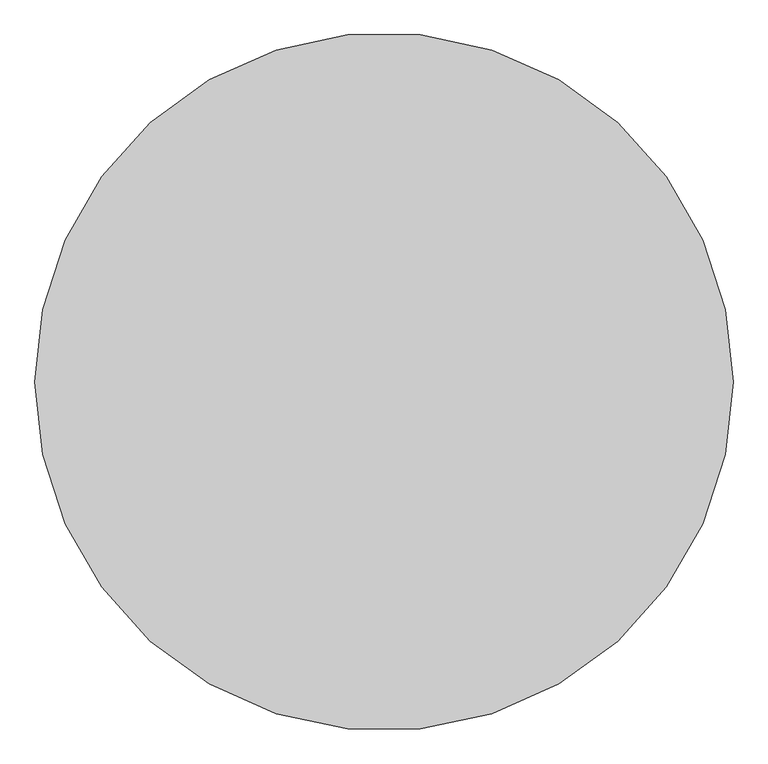
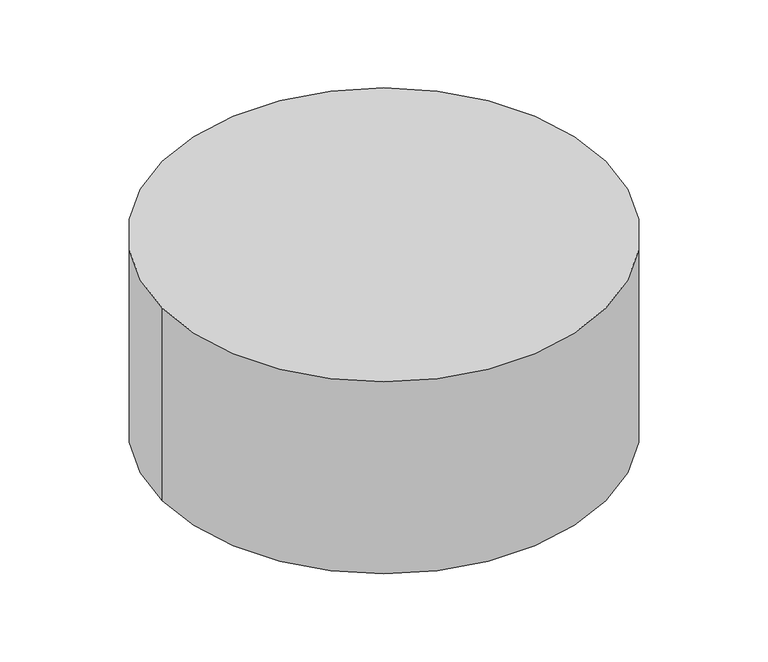
"""IFC4 building model written with IfcOpenShell, lengths in millimetres: proxy geometry, 일반 모델 2 : 일반 모델 2."""

from ifc_helpers import new_model, si_unit, point, frame, frame_2d, origin, place, context, project, spatial, circle_curve, trimmed, segment, composite_curve, outline, extrude, source, transform, mapped, element, save


def generic_models_93d6a0fc(model_context):
    return source(origin(), model_context, "Body", "SweptSolid", [
        extrude(outline(composite_curve([segment(trimmed(circle_curve(frame_2d((-3410.7544062, 1589.1761456)), 1200.0), [point((-4610.7544062, 1589.1761456))], [point((-2210.7544062, 1589.1761456))], False, "CARTESIAN"), True, "CONTINUOUS"), segment(trimmed(circle_curve(frame_2d((-3410.7544062, 1589.1761456)), 1200.0), [point((-2210.7544062, 1589.1761456))], [point((-4610.7544062, 1589.1761456))], False, "CARTESIAN"), True, "CONTINUOUS")], self_intersect=False)), frame((0.0, 0.0, 250.0), z_axis=(0.0, 0.0, 1.0), x_axis=(1.0, 0.0, 0.0)), (0.0, 0.0, 1.0), 1100.0),
    ])


if __name__ == "__main__":
    model = new_model("IFC4")
    model_context = context("Model", 3, world=origin())
    ifc_project = project(units=[si_unit("LENGTHUNIT", "METRE", prefix="MILLI")], contexts=[model_context])
    site = spatial("IfcSite", under=ifc_project)
    building = spatial("IfcBuilding", under=site)
    placement = place(None, origin())
    generic_models_shape = generic_models_93d6a0fc(model_context)
    element("IfcBuildingElementProxy", 1, Name="일반 모델 2 : 일반 모델 2", ObjectType="일반 모델 2 : 일반 모델 2", at=placement, inside=building, context=model_context, shape_type="MappedRepresentation", body=[
        mapped(generic_models_shape, transform((0.0, 0.0, 0.0), x_axis=(1.0, 0.0, 0.0), y_axis=(0.0, 1.0, 0.0), z_axis=(0.0, 0.0, 1.0))),
    ])
    save(model, "model.ifc")

# Revit data of these elements
# Type "일반 모델 2 : 일반 모델 2"
#   Type Mark = "StepLED.L.B.2"
# Element 1 (IfcBuildingElementProxy, "일반 모델 2 : 일반 모델 2")
#   Materials on its faces: "led_g"
# Materials
#   "led_g": class "일반", colour RGB 0 255 0, transparency 1, Cost = 0
